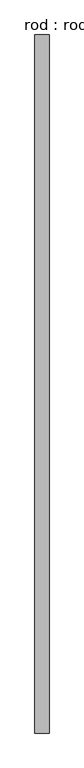
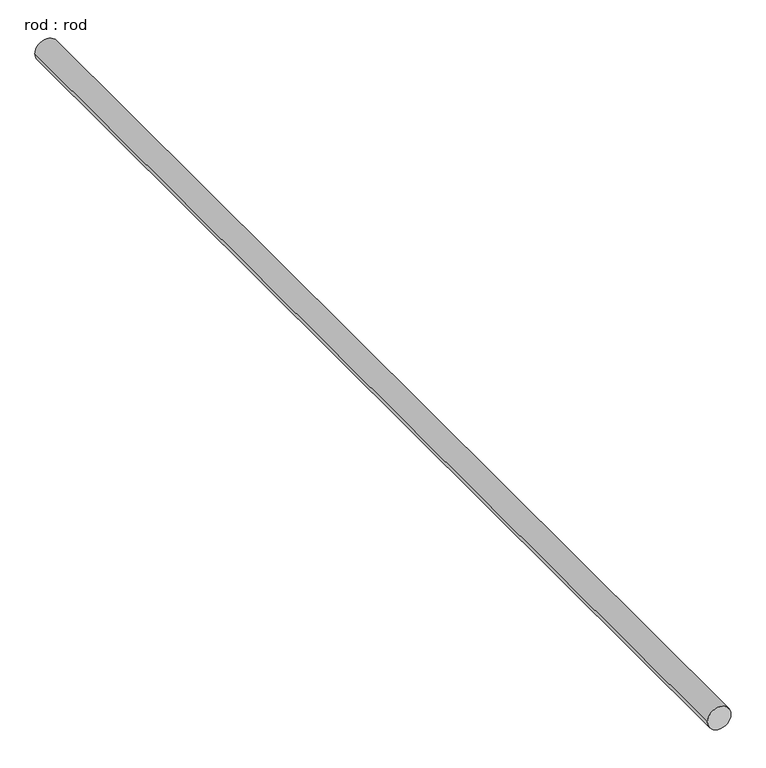
"""IFC4 building model written with IfcOpenShell, lengths in millimetres: proxy geometry, rod : rod."""

import ifcopenshell
import ifcopenshell.guid

model = None  # the IFC model being written
_history = None  # IfcOwnerHistory: only IFC2X3 demands one
_inside = {}  # id of a spatial element -> (the spatial element, [elements in it])
_under = {}  # id of a project, library or spatial element -> (it, [spatial elements below it])
_declared = {}  # id of a project -> (the project, [libraries it declares])
_typed = {}  # id of a type object -> (the type object, [elements of that type])
_made_of = {}  # id of a material, layer set ... -> (it, [elements and type objects made of it])


def new_model(schema):
    """Start an empty IFC model of exactly this schema.

    Asked for "IFC4X3", IfcOpenShell would pick the latest addendum, in which some entities
    have other attributes; the version numbers below select the first issue.
    IFC2X3 requires an IfcOwnerHistory on every rooted entity: one is made here for all.
    """
    global model, _history
    if schema == "IFC4X3":
        model = ifcopenshell.file(schema_version=(4, 3, 0, 0))
    else:
        model = ifcopenshell.file(schema=schema)
    _inside.clear()
    _under.clear()
    _declared.clear()
    _typed.clear()
    _made_of.clear()
    _history = None
    if model.schema == "IFC2X3":
        org = make("IfcOrganization", Name="unknown")
        user = make(
            "IfcPersonAndOrganization",
            ThePerson=make("IfcPerson", FamilyName="unknown"),
            TheOrganization=org,
        )
        app = make(
            "IfcApplication",
            ApplicationDeveloper=org,
            Version="unknown",
            ApplicationFullName="unknown",
            ApplicationIdentifier="unknown",
        )
        _history = make(
            "IfcOwnerHistory",
            OwningUser=user,
            OwningApplication=app,
            ChangeAction="ADDED",
            CreationDate=0,
        )
    return model


def make(cls, **values):
    """One entity of the class cls with the attributes given. An attribute that is None is left unset."""
    return model.create_entity(
        cls, **{name: value for name, value in values.items() if value is not None}
    )


def rooted(cls, **values):
    """An entity with a GlobalId (a new one), such as an element, a storey or a relation."""
    return make(cls, GlobalId=ifcopenshell.guid.new(), OwnerHistory=_history, **values)


def si_unit(unit_type, name, prefix=None):
    """IfcSIUnit, for example si_unit("LENGTHUNIT", "METRE", prefix="MILLI")."""
    return make("IfcSIUnit", UnitType=unit_type, Prefix=prefix, Name=name)


def assignment(units):
    """IfcUnitAssignment: the units of a project."""
    return None if units is None else make("IfcUnitAssignment", Units=units)


def point(xyz):
    """IfcCartesianPoint."""
    return None if xyz is None else make("IfcCartesianPoint", Coordinates=xyz)


def direction(xyz):
    """IfcDirection."""
    return None if xyz is None else make("IfcDirection", DirectionRatios=xyz)


def frame(location, z_axis=None, x_axis=None):
    """IfcAxis2Placement3D, a coordinate frame: its origin and axes. An axis left out is left unset."""
    return make(
        "IfcAxis2Placement3D",
        Location=point(location),
        Axis=direction(z_axis),
        RefDirection=direction(x_axis),
    )


def frame_2d(location, x_axis=None):
    """IfcAxis2Placement2D, a coordinate frame in the plane: its origin and x axis."""
    return make(
        "IfcAxis2Placement2D", Location=point(location), RefDirection=direction(x_axis)
    )


def origin():
    """The frame at (0, 0, 0) with its axes left unset."""
    return frame((0.0, 0.0, 0.0))


def place(relative_to, where):
    """IfcLocalPlacement: puts the frame where relative to a parent placement (None: the world)."""
    return make(
        "IfcLocalPlacement", PlacementRelTo=relative_to, RelativePlacement=where
    )


def context(
    kind, dimensions, precision=None, world=None, true_north=None, identifier=None
):
    """IfcGeometricRepresentationContext, for example the 3D "Model" context."""
    return make(
        "IfcGeometricRepresentationContext",
        ContextIdentifier=identifier,
        ContextType=kind,
        CoordinateSpaceDimension=dimensions,
        Precision=precision,
        WorldCoordinateSystem=world,
        TrueNorth=true_north,
    )


def project(units=None, contexts=None):
    """IfcProject with its units and contexts."""
    return rooted(
        "IfcProject",
        Name="project",
        RepresentationContexts=contexts,
        UnitsInContext=assignment(units),
    )


def spatial(cls, under=None, at=None, **own):
    """A site, building, storey or space (cls), placed at a placement, below another one or the project."""
    s = rooted(cls, ObjectPlacement=at, **own)
    if under is not None:
        _under.setdefault(under.id(), (under, []))[1].append(s)
    return s


def circle_curve(where, radius):
    """IfcCircle in the frame where."""
    return make("IfcCircle", Position=where, Radius=radius)


def trimmed(basis, trim1, trim2, sense, master):
    """IfcTrimmedCurve: the piece of a basis curve between two trims."""
    return make(
        "IfcTrimmedCurve",
        BasisCurve=basis,
        Trim1=trim1,
        Trim2=trim2,
        SenseAgreement=sense,
        MasterRepresentation=master,
    )


def segment(curve, same_sense, transition):
    """IfcCompositeCurveSegment."""
    return make(
        "IfcCompositeCurveSegment",
        Transition=transition,
        SameSense=same_sense,
        ParentCurve=curve,
    )


def composite_curve(segments, self_intersect=None):
    """IfcCompositeCurve: segments joined end to end."""
    return make("IfcCompositeCurve", Segments=segments, SelfIntersect=self_intersect)


def outline(outer, holes=None, kind="AREA"):
    """IfcArbitraryClosedProfileDef: a profile drawn as a closed curve; with holes, ...WithVoids."""
    if holes is None:
        return make("IfcArbitraryClosedProfileDef", ProfileType=kind, OuterCurve=outer)
    return make(
        "IfcArbitraryProfileDefWithVoids",
        ProfileType=kind,
        OuterCurve=outer,
        InnerCurves=holes,
    )


def extrude(swept, where, along, depth):
    """IfcExtrudedAreaSolid: the profile swept, set in the frame where, extruded along a direction by depth."""
    return make(
        "IfcExtrudedAreaSolid",
        SweptArea=swept,
        Position=where,
        ExtrudedDirection=direction(along),
        Depth=depth,
    )


def shape(context_of_items, identifier, shape_type, items):
    """IfcShapeRepresentation: the items that make up one representation, for example the "Body"."""
    return make(
        "IfcShapeRepresentation",
        ContextOfItems=context_of_items,
        RepresentationIdentifier=identifier,
        RepresentationType=shape_type,
        Items=items,
    )


def source(mapping_origin, context_of_items, identifier, shape_type, items):
    """IfcRepresentationMap: a shape defined once, which mapped items show again and again."""
    return make(
        "IfcRepresentationMap",
        MappingOrigin=mapping_origin,
        MappedRepresentation=shape(context_of_items, identifier, shape_type, items),
    )


def transform(
    local_origin,
    x_axis=None,
    y_axis=None,
    z_axis=None,
    scale=None,
    scale2=None,
    scale3=None,
    uniform=True,
):
    """IfcCartesianTransformationOperator3D, or its non-uniform kind. x_axis, y_axis, z_axis: its Axis1, 2, 3."""
    if uniform:
        return make(
            "IfcCartesianTransformationOperator3D",
            Axis1=direction(x_axis),
            Axis2=direction(y_axis),
            LocalOrigin=point(local_origin),
            Scale=scale,
            Axis3=direction(z_axis),
        )
    return make(
        "IfcCartesianTransformationOperator3DnonUniform",
        Axis1=direction(x_axis),
        Axis2=direction(y_axis),
        LocalOrigin=point(local_origin),
        Scale=scale,
        Axis3=direction(z_axis),
        Scale2=scale2,
        Scale3=scale3,
    )


def mapped(mapping_source, mapping_target):
    """IfcMappedItem: shows the shape of a source again, moved by a transform."""
    return make(
        "IfcMappedItem", MappingSource=mapping_source, MappingTarget=mapping_target
    )


def made_of(thing, what):
    """Note that an element or type object is made of a material, layer set ...; save() writes the relation."""
    if what is not None:
        _made_of.setdefault(what.id(), (what, []))[1].append(thing)
    return thing


def element(
    cls,
    number,
    at=None,
    inside=None,
    cuts=None,
    type_object=None,
    material=None,
    context=None,
    identifier="Body",
    shape_type=None,
    held_by="IfcProductDefinitionShape",
    body=None,
    shapes=None,
    **own,
):
    """One element of the class cls, such as IfcWall. Its Tag is "e" and its number.

    at: its placement. inside: the storey or other place that contains it. cuts: it is an
    opening in that element (IfcRelVoidsElement). A single representation is given by context,
    identifier, shape_type and body (its items); several are given by shapes. held_by: the class
    of the entity that holds the representations. save() writes the other relations.
    """
    e = rooted(cls, Tag="e%d" % number, ObjectPlacement=at, **own)
    if body is not None:
        shapes = [shape(context, identifier, shape_type, body)]
    if shapes is not None:
        e.Representation = make(held_by, Representations=shapes)
    if inside is not None:
        _inside.setdefault(inside.id(), (inside, []))[1].append(e)
    if cuts is not None:
        rooted(
            "IfcRelVoidsElement", RelatingBuildingElement=cuts, RelatedOpeningElement=e
        )
    if type_object is not None:
        _typed.setdefault(type_object.id(), (type_object, []))[1].append(e)
    return made_of(e, material)


def aggregate(whole, parts):
    """IfcRelAggregates: a whole, such as a stair, and the parts it consists of."""
    return rooted("IfcRelAggregates", RelatingObject=whole, RelatedObjects=parts)


def save(model, path):
    """Write the relations noted so far, then the file.

    IfcRelAggregates (storeys below a building ...), IfcRelContainedInSpatialStructure (elements
    in a storey), IfcRelDefinesByType, IfcRelAssociatesMaterial and IfcRelDeclares: one each for
    every whole, place, type object, material and project.
    """
    for whole, parts in _under.values():
        aggregate(whole, parts)
    for where, things in _inside.values():
        rooted(
            "IfcRelContainedInSpatialStructure",
            RelatedElements=things,
            RelatingStructure=where,
        )
    for kind, things in _typed.values():
        rooted("IfcRelDefinesByType", RelatedObjects=things, RelatingType=kind)
    for what, things in _made_of.values():
        rooted("IfcRelAssociatesMaterial", RelatedObjects=things, RelatingMaterial=what)
    for by, libraries in _declared.values():
        rooted("IfcRelDeclares", RelatingContext=by, RelatedDefinitions=libraries)
    model.write(path)


def rod_rod_f18bf7d2(model_context):
    return source(origin(), model_context, "Body", "SweptSolid", [
        extrude(outline(composite_curve([segment(trimmed(circle_curve(frame_2d((0.0108462, 0.0)), 200.0), [point((0.0108462, 200.0))], [point((0.0108462, -200.0))], False, "CARTESIAN"), True, "CONTINUOUS"), segment(trimmed(circle_curve(frame_2d((0.0108462, 0.0)), 200.0), [point((0.0108462, -200.0))], [point((0.0108462, 200.0))], False, "CARTESIAN"), True, "CONTINUOUS")], self_intersect=False)), frame((0.0, -5804.5928132, 0.0), z_axis=(0.0, 1.0, 0.0), x_axis=(0.0, 0.0, 1.0)), (0.0, 0.0, 1.0), 19794.6428571),
    ])


if __name__ == "__main__":
    model = new_model("IFC4")
    model_context = context("Model", 3, world=origin())
    ifc_project = project(units=[si_unit("LENGTHUNIT", "METRE", prefix="MILLI")], contexts=[model_context])
    site = spatial("IfcSite", under=ifc_project)
    building = spatial("IfcBuilding", under=site)
    placement = place(None, origin())
    rod_rod_shape = rod_rod_f18bf7d2(model_context)
    element("IfcBuildingElementProxy", 1, Name="rod : rod", ObjectType="rod : rod", at=placement, inside=building, context=model_context, shape_type="MappedRepresentation", body=[
        mapped(rod_rod_shape, transform((0.0, 0.0, 0.0), x_axis=(1.0, 0.0, 0.0), y_axis=(0.0, 1.0, 0.0), z_axis=(0.0, 0.0, 1.0))),
    ])
    save(model, "model.ifc")

# Revit data of these elements
# Type "rod : rod"
#   Default Elevation = 0
